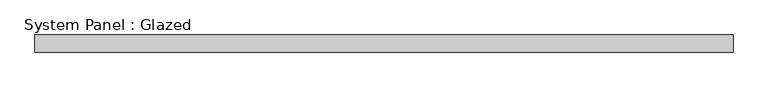
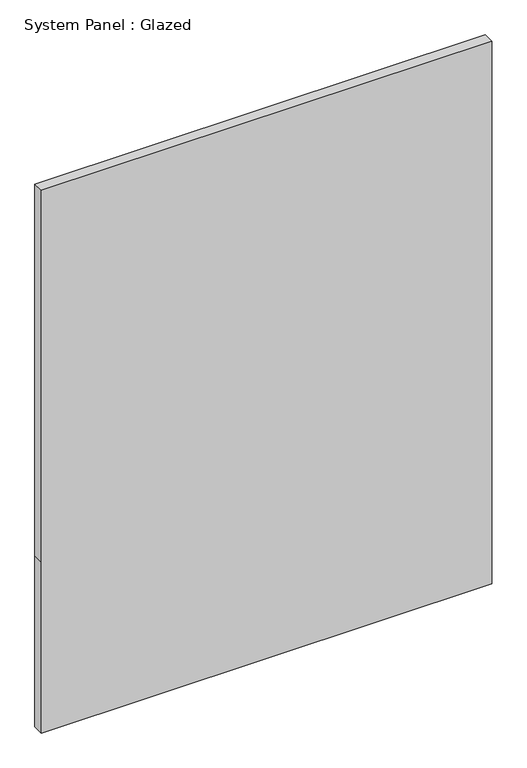
"""IFC4 building model written with IfcOpenShell, lengths in millimetres: plate geometry, System Panel : Glazed."""

from ifc_helpers import new_model, si_unit, frame, origin, place, context, project, spatial, polyline, outline, extrude, source, transform, mapped, element, save


def system_panel_glazed_a9001392(model_context):
    return source(origin(), model_context, "Body", "SweptSolid", [
        extrude(outline(polyline([(0.0, -505.8833333), (0.0, 505.8833333), (406.4, 505.8833333), (1289.05, 505.8833333), (1289.05, -505.8833333), (406.4, -505.8833333), (0.0, -505.8833333)])), frame((0.0, 19.05, 0.0), z_axis=(0.0, 1.0, 0.0), x_axis=(0.0, 0.0, 1.0)), (0.0, 0.0, 1.0), 25.4),
    ])


if __name__ == "__main__":
    model = new_model("IFC4")
    model_context = context("Model", 3, world=origin())
    ifc_project = project(units=[si_unit("LENGTHUNIT", "METRE", prefix="MILLI")], contexts=[model_context])
    site = spatial("IfcSite", under=ifc_project)
    building = spatial("IfcBuilding", under=site)
    placement = place(None, origin())
    system_panel_glazed_shape = system_panel_glazed_a9001392(model_context)
    element("IfcPlate", 1, ObjectType="System Panel : Glazed", at=placement, inside=building, context=model_context, shape_type="MappedRepresentation", body=[
        mapped(system_panel_glazed_shape, transform((0.0, 0.0, 0.0), x_axis=(1.0, 0.0, 0.0), y_axis=(0.0, 1.0, 0.0), z_axis=(0.0, 0.0, 1.0))),
    ])
    save(model, "model.ifc")

# Revit data of these elements
# Type "System Panel : Glazed"
#   Analytic Construction = "1/8 in Pilkington single glazing"
#   Visual Light Transmittance = 0.9
#   Solar Heat Gain Coefficient = 0.86
#   Heat Transfer Coefficient (U) = 1.18115 BTU/(h·ft²·°F)
# Element 1 (IfcPlate, "System Panel : Glazed")
#   Materials on its faces: "Glass, Clear Glazing"
# Materials
#   "Glass, Clear Glazing": class "Glass", colour RGB 245 245 243, transparency 1, Description = "Clear glazing", Cost = 0
